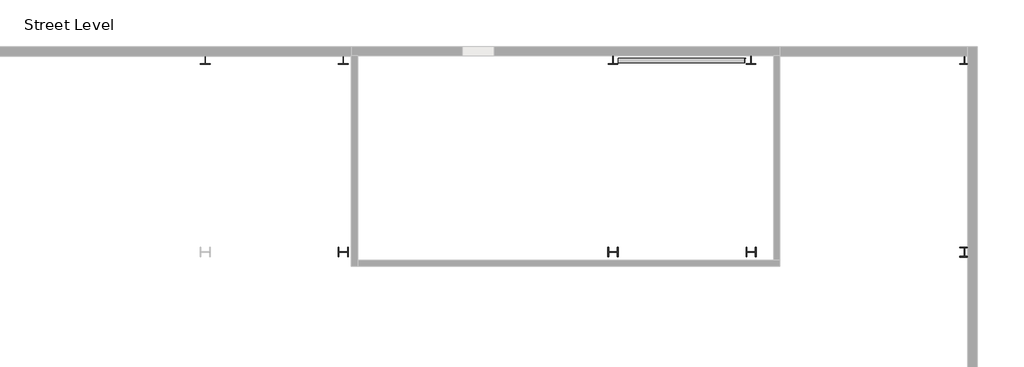
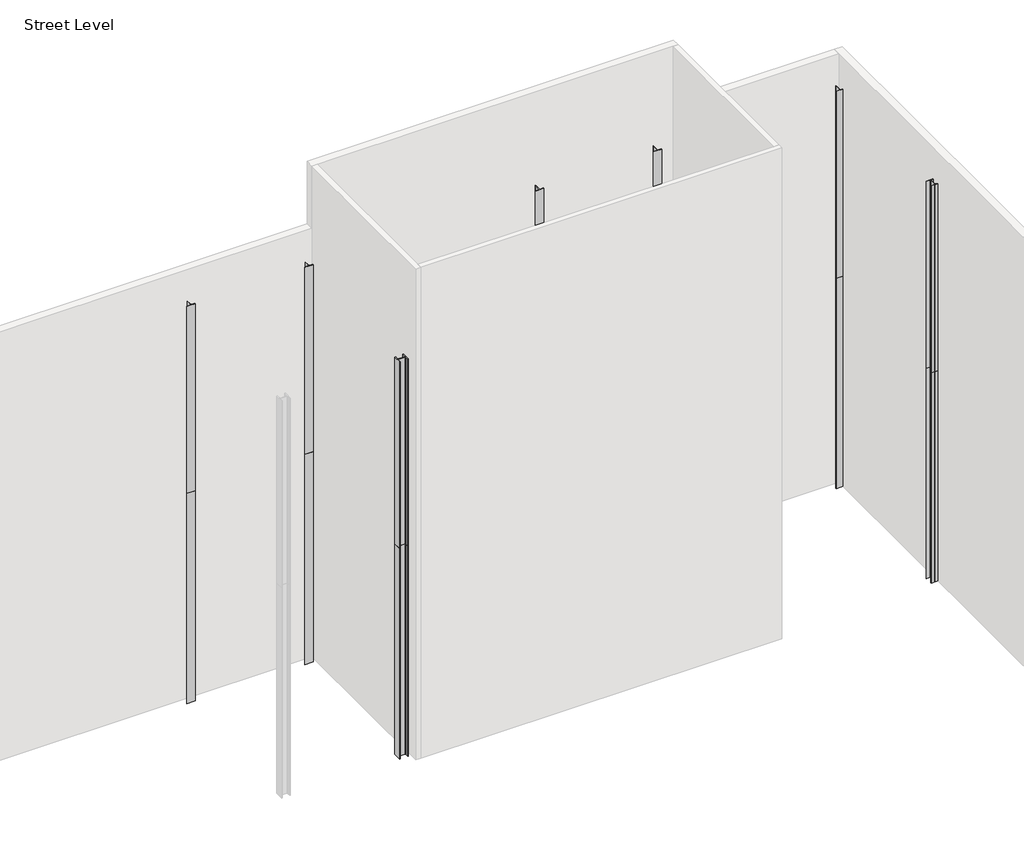
# One storey, part 3 of 3: 9 columns, 1 member.
"""IFC4 building model written with IfcOpenShell, lengths in millimetres."""

import ifcopenshell
import ifcopenshell.guid

model = None  # the IFC model being written
_history = None  # IfcOwnerHistory: only IFC2X3 demands one
_inside = {}  # id of a spatial element -> (the spatial element, [elements in it])
_under = {}  # id of a project, library or spatial element -> (it, [spatial elements below it])
_declared = {}  # id of a project -> (the project, [libraries it declares])
_typed = {}  # id of a type object -> (the type object, [elements of that type])
_made_of = {}  # id of a material, layer set ... -> (it, [elements and type objects made of it])


def new_model(schema):
    """Start an empty IFC model of exactly this schema.

    Asked for "IFC4X3", IfcOpenShell would pick the latest addendum, in which some entities
    have other attributes; the version numbers below select the first issue.
    IFC2X3 requires an IfcOwnerHistory on every rooted entity: one is made here for all.
    """
    global model, _history
    if schema == "IFC4X3":
        model = ifcopenshell.file(schema_version=(4, 3, 0, 0))
    else:
        model = ifcopenshell.file(schema=schema)
    _inside.clear()
    _under.clear()
    _declared.clear()
    _typed.clear()
    _made_of.clear()
    _history = None
    if model.schema == "IFC2X3":
        org = make("IfcOrganization", Name="unknown")
        user = make(
            "IfcPersonAndOrganization",
            ThePerson=make("IfcPerson", FamilyName="unknown"),
            TheOrganization=org,
        )
        app = make(
            "IfcApplication",
            ApplicationDeveloper=org,
            Version="unknown",
            ApplicationFullName="unknown",
            ApplicationIdentifier="unknown",
        )
        _history = make(
            "IfcOwnerHistory",
            OwningUser=user,
            OwningApplication=app,
            ChangeAction="ADDED",
            CreationDate=0,
        )
    return model


def make(cls, **values):
    """One entity of the class cls with the attributes given. An attribute that is None is left unset."""
    return model.create_entity(
        cls, **{name: value for name, value in values.items() if value is not None}
    )


def rooted(cls, **values):
    """An entity with a GlobalId (a new one), such as an element, a storey or a relation."""
    return make(cls, GlobalId=ifcopenshell.guid.new(), OwnerHistory=_history, **values)


def si_unit(unit_type, name, prefix=None):
    """IfcSIUnit, for example si_unit("LENGTHUNIT", "METRE", prefix="MILLI")."""
    return make("IfcSIUnit", UnitType=unit_type, Prefix=prefix, Name=name)


def assignment(units):
    """IfcUnitAssignment: the units of a project."""
    return None if units is None else make("IfcUnitAssignment", Units=units)


def point(xyz):
    """IfcCartesianPoint."""
    return None if xyz is None else make("IfcCartesianPoint", Coordinates=xyz)


def direction(xyz):
    """IfcDirection."""
    return None if xyz is None else make("IfcDirection", DirectionRatios=xyz)


def frame(location, z_axis=None, x_axis=None):
    """IfcAxis2Placement3D, a coordinate frame: its origin and axes. An axis left out is left unset."""
    return make(
        "IfcAxis2Placement3D",
        Location=point(location),
        Axis=direction(z_axis),
        RefDirection=direction(x_axis),
    )


def frame_2d(location, x_axis=None):
    """IfcAxis2Placement2D, a coordinate frame in the plane: its origin and x axis."""
    return make(
        "IfcAxis2Placement2D", Location=point(location), RefDirection=direction(x_axis)
    )


def origin():
    """The frame at (0, 0, 0) with its axes left unset."""
    return frame((0.0, 0.0, 0.0))


def place(relative_to, where):
    """IfcLocalPlacement: puts the frame where relative to a parent placement (None: the world)."""
    return make(
        "IfcLocalPlacement", PlacementRelTo=relative_to, RelativePlacement=where
    )


def context(
    kind, dimensions, precision=None, world=None, true_north=None, identifier=None
):
    """IfcGeometricRepresentationContext, for example the 3D "Model" context."""
    return make(
        "IfcGeometricRepresentationContext",
        ContextIdentifier=identifier,
        ContextType=kind,
        CoordinateSpaceDimension=dimensions,
        Precision=precision,
        WorldCoordinateSystem=world,
        TrueNorth=true_north,
    )


def project(units=None, contexts=None):
    """IfcProject with its units and contexts."""
    return rooted(
        "IfcProject",
        Name="project",
        RepresentationContexts=contexts,
        UnitsInContext=assignment(units),
    )


def spatial(cls, under=None, at=None, **own):
    """A site, building, storey or space (cls), placed at a placement, below another one or the project."""
    s = rooted(cls, ObjectPlacement=at, **own)
    if under is not None:
        _under.setdefault(under.id(), (under, []))[1].append(s)
    return s


def polyline(points):
    """IfcPolyline through the points."""
    return make("IfcPolyline", Points=[point(p) for p in points])


def circle_curve(where, radius):
    """IfcCircle in the frame where."""
    return make("IfcCircle", Position=where, Radius=radius)


def trimmed(basis, trim1, trim2, sense, master):
    """IfcTrimmedCurve: the piece of a basis curve between two trims."""
    return make(
        "IfcTrimmedCurve",
        BasisCurve=basis,
        Trim1=trim1,
        Trim2=trim2,
        SenseAgreement=sense,
        MasterRepresentation=master,
    )


def segment(curve, same_sense, transition):
    """IfcCompositeCurveSegment."""
    return make(
        "IfcCompositeCurveSegment",
        Transition=transition,
        SameSense=same_sense,
        ParentCurve=curve,
    )


def composite_curve(segments, self_intersect=None):
    """IfcCompositeCurve: segments joined end to end."""
    return make("IfcCompositeCurve", Segments=segments, SelfIntersect=self_intersect)


def outline(outer, holes=None, kind="AREA"):
    """IfcArbitraryClosedProfileDef: a profile drawn as a closed curve; with holes, ...WithVoids."""
    if holes is None:
        return make("IfcArbitraryClosedProfileDef", ProfileType=kind, OuterCurve=outer)
    return make(
        "IfcArbitraryProfileDefWithVoids",
        ProfileType=kind,
        OuterCurve=outer,
        InnerCurves=holes,
    )


def extrude(swept, where, along, depth):
    """IfcExtrudedAreaSolid: the profile swept, set in the frame where, extruded along a direction by depth."""
    return make(
        "IfcExtrudedAreaSolid",
        SweptArea=swept,
        Position=where,
        ExtrudedDirection=direction(along),
        Depth=depth,
    )


def shape(context_of_items, identifier, shape_type, items):
    """IfcShapeRepresentation: the items that make up one representation, for example the "Body"."""
    return make(
        "IfcShapeRepresentation",
        ContextOfItems=context_of_items,
        RepresentationIdentifier=identifier,
        RepresentationType=shape_type,
        Items=items,
    )


def source(mapping_origin, context_of_items, identifier, shape_type, items):
    """IfcRepresentationMap: a shape defined once, which mapped items show again and again."""
    return make(
        "IfcRepresentationMap",
        MappingOrigin=mapping_origin,
        MappedRepresentation=shape(context_of_items, identifier, shape_type, items),
    )


def transform(
    local_origin,
    x_axis=None,
    y_axis=None,
    z_axis=None,
    scale=None,
    scale2=None,
    scale3=None,
    uniform=True,
):
    """IfcCartesianTransformationOperator3D, or its non-uniform kind. x_axis, y_axis, z_axis: its Axis1, 2, 3."""
    if uniform:
        return make(
            "IfcCartesianTransformationOperator3D",
            Axis1=direction(x_axis),
            Axis2=direction(y_axis),
            LocalOrigin=point(local_origin),
            Scale=scale,
            Axis3=direction(z_axis),
        )
    return make(
        "IfcCartesianTransformationOperator3DnonUniform",
        Axis1=direction(x_axis),
        Axis2=direction(y_axis),
        LocalOrigin=point(local_origin),
        Scale=scale,
        Axis3=direction(z_axis),
        Scale2=scale2,
        Scale3=scale3,
    )


def mapped(mapping_source, mapping_target):
    """IfcMappedItem: shows the shape of a source again, moved by a transform."""
    return make(
        "IfcMappedItem", MappingSource=mapping_source, MappingTarget=mapping_target
    )


def made_of(thing, what):
    """Note that an element or type object is made of a material, layer set ...; save() writes the relation."""
    if what is not None:
        _made_of.setdefault(what.id(), (what, []))[1].append(thing)
    return thing


def element(
    cls,
    number,
    at=None,
    inside=None,
    cuts=None,
    type_object=None,
    material=None,
    context=None,
    identifier="Body",
    shape_type=None,
    held_by="IfcProductDefinitionShape",
    body=None,
    shapes=None,
    **own,
):
    """One element of the class cls, such as IfcWall. Its Tag is "e" and its number.

    at: its placement. inside: the storey or other place that contains it. cuts: it is an
    opening in that element (IfcRelVoidsElement). A single representation is given by context,
    identifier, shape_type and body (its items); several are given by shapes. held_by: the class
    of the entity that holds the representations. save() writes the other relations.
    """
    e = rooted(cls, Tag="e%d" % number, ObjectPlacement=at, **own)
    if body is not None:
        shapes = [shape(context, identifier, shape_type, body)]
    if shapes is not None:
        e.Representation = make(held_by, Representations=shapes)
    if inside is not None:
        _inside.setdefault(inside.id(), (inside, []))[1].append(e)
    if cuts is not None:
        rooted(
            "IfcRelVoidsElement", RelatingBuildingElement=cuts, RelatedOpeningElement=e
        )
    if type_object is not None:
        _typed.setdefault(type_object.id(), (type_object, []))[1].append(e)
    return made_of(e, material)


def aggregate(whole, parts):
    """IfcRelAggregates: a whole, such as a stair, and the parts it consists of."""
    return rooted("IfcRelAggregates", RelatingObject=whole, RelatedObjects=parts)


def save(model, path):
    """Write the relations noted so far, then the file.

    IfcRelAggregates (storeys below a building ...), IfcRelContainedInSpatialStructure (elements
    in a storey), IfcRelDefinesByType, IfcRelAssociatesMaterial and IfcRelDeclares: one each for
    every whole, place, type object, material and project.
    """
    for whole, parts in _under.values():
        aggregate(whole, parts)
    for where, things in _inside.values():
        rooted(
            "IfcRelContainedInSpatialStructure",
            RelatedElements=things,
            RelatingStructure=where,
        )
    for kind, things in _typed.values():
        rooted("IfcRelDefinesByType", RelatedObjects=things, RelatingType=kind)
    for what, things in _made_of.values():
        rooted("IfcRelAssociatesMaterial", RelatedObjects=things, RelatingMaterial=what)
    for by, libraries in _declared.values():
        rooted("IfcRelDeclares", RelatingContext=by, RelatedDefinitions=libraries)
    model.write(path)


def l_angle_l6x6x3_8_1e5b70da(model_context):
    return source(origin(), model_context, "Body", "SweptSolid", [
        extrude(outline(composite_curve([segment(polyline([(41.148, 41.148), (41.148, -111.252)]), True, "CONTINUOUS"), segment(trimmed(circle_curve(frame_2d((41.148, -101.727)), 9.525), [point((41.148, -111.252))], [point((31.623, -101.727))], False, "CARTESIAN"), True, "CONTINUOUS"), segment(polyline([(31.623, -101.727), (31.623, 22.098)]), True, "CONTINUOUS"), segment(trimmed(circle_curve(frame_2d((22.098, 22.098)), 9.525), [point((31.623, 22.098))], [point((22.098, 31.623))], True, "CARTESIAN"), True, "CONTINUOUS"), segment(polyline([(22.098, 31.623), (-101.727, 31.623)]), True, "CONTINUOUS"), segment(trimmed(circle_curve(frame_2d((-101.727, 41.148)), 9.525), [point((-101.727, 31.623))], [point((-111.252, 41.148))], False, "CARTESIAN"), True, "CONTINUOUS"), segment(polyline([(-111.252, 41.148), (41.148, 41.148)]), True, "CONTINUOUS")], self_intersect=False)), frame((-2053.4214347, 0.0, 0.0), z_axis=(1.0, 0.0, 0.0), x_axis=(0.0, 1.0, 0.0)), (0.0, 0.0, 1.0), 4092.1699392),
    ])


model = new_model("IFC4")

# Units and contexts
model_context = context("Model", 3, world=origin())
ifc_project = project(units=[si_unit("LENGTHUNIT", "METRE", prefix="MILLI")], contexts=[model_context])

# Site, building, storey
site = spatial("IfcSite", under=ifc_project)
building = spatial("IfcBuilding", under=site)
storey = spatial("IfcBuildingStorey", under=building, Name="Street Level", Elevation=-914.4)

# Columns
placement = place(None, origin())
element("IfcColumn", 1, ObjectType="W-Wide Flange-Column : W12X87", at=placement, inside=storey, context=model_context, shape_type="SweptSolid", body=[
    extrude(outline(composite_curve([segment(polyline([(-5274.2622732, 2940.2315304), (-5294.8362732, 2940.2315304), (-5294.8362732, 3065.0725304)]), True, "CONTINUOUS"), segment(trimmed(circle_curve(frame_2d((-5317.1247732, 3065.0725304)), 22.2885), [point((-5294.8362732, 3065.0725304))], [point((-5317.1247732, 3087.3610304))], True, "CARTESIAN"), True, "CONTINUOUS"), segment(polyline([(-5317.1247732, 3087.3610304), (-5548.8997732, 3087.3610304)]), True, "CONTINUOUS"), segment(trimmed(circle_curve(frame_2d((-5548.8997732, 3065.0725304)), 22.2885), [point((-5548.8997732, 3087.3610304))], [point((-5571.1882732, 3065.0725304))], True, "CARTESIAN"), True, "CONTINUOUS"), segment(polyline([(-5571.1882732, 3065.0725304), (-5571.1882732, 2940.2315304), (-5591.7622732, 2940.2315304), (-5591.7622732, 3247.5715304), (-5571.1882732, 3247.5715304), (-5571.1882732, 3122.7305304)]), True, "CONTINUOUS"), segment(trimmed(circle_curve(frame_2d((-5548.8997732, 3122.7305304)), 22.2885), [point((-5571.1882732, 3122.7305304))], [point((-5548.8997732, 3100.4420304))], True, "CARTESIAN"), True, "CONTINUOUS"), segment(polyline([(-5548.8997732, 3100.4420304), (-5317.1247732, 3100.4420304)]), True, "CONTINUOUS"), segment(trimmed(circle_curve(frame_2d((-5317.1247732, 3122.7305304)), 22.2885), [point((-5317.1247732, 3100.4420304))], [point((-5294.8362732, 3122.7305304))], True, "CARTESIAN"), True, "CONTINUOUS"), segment(polyline([(-5294.8362732, 3122.7305304), (-5294.8362732, 3247.5715304), (-5274.2622732, 3247.5715304), (-5274.2622732, 2940.2315304)]), True, "CONTINUOUS")], self_intersect=False)), frame((0.0, 0.0, 7315.2), z_axis=(0.0, 0.0, 1.0), x_axis=(1.0, 0.0, 0.0)), (0.0, 0.0, 1.0), 7315.2),
    extrude(outline(composite_curve([segment(polyline([(-5274.2622732, 2940.2315304), (-5294.8362732, 2940.2315304), (-5294.8362732, 3065.0725304)]), True, "CONTINUOUS"), segment(trimmed(circle_curve(frame_2d((-5317.1247732, 3065.0725304)), 22.2885), [point((-5294.8362732, 3065.0725304))], [point((-5317.1247732, 3087.3610304))], True, "CARTESIAN"), True, "CONTINUOUS"), segment(polyline([(-5317.1247732, 3087.3610304), (-5548.8997732, 3087.3610304)]), True, "CONTINUOUS"), segment(trimmed(circle_curve(frame_2d((-5548.8997732, 3065.0725304)), 22.2885), [point((-5548.8997732, 3087.3610304))], [point((-5571.1882732, 3065.0725304))], True, "CARTESIAN"), True, "CONTINUOUS"), segment(polyline([(-5571.1882732, 3065.0725304), (-5571.1882732, 2940.2315304), (-5591.7622732, 2940.2315304), (-5591.7622732, 3247.5715304), (-5571.1882732, 3247.5715304), (-5571.1882732, 3122.7305304)]), True, "CONTINUOUS"), segment(trimmed(circle_curve(frame_2d((-5548.8997732, 3122.7305304)), 22.2885), [point((-5571.1882732, 3122.7305304))], [point((-5548.8997732, 3100.4420304))], True, "CARTESIAN"), True, "CONTINUOUS"), segment(polyline([(-5548.8997732, 3100.4420304), (-5317.1247732, 3100.4420304)]), True, "CONTINUOUS"), segment(trimmed(circle_curve(frame_2d((-5317.1247732, 3122.7305304)), 22.2885), [point((-5317.1247732, 3100.4420304))], [point((-5294.8362732, 3122.7305304))], True, "CARTESIAN"), True, "CONTINUOUS"), segment(polyline([(-5294.8362732, 3122.7305304), (-5294.8362732, 3247.5715304), (-5274.2622732, 3247.5715304), (-5274.2622732, 2940.2315304)]), True, "CONTINUOUS")], self_intersect=False)), frame((0.0, 0.0, -914.4), z_axis=(0.0, 0.0, 1.0), x_axis=(1.0, 0.0, 0.0)), (0.0, 0.0, 1.0), 8229.6),
])
element("IfcColumn", 2, ObjectType="W-Wide Flange-Column : W12X87", at=placement, inside=storey, context=model_context, shape_type="SweptSolid", body=[
    extrude(outline(composite_curve([segment(polyline([(3260.1377268, 2940.2315304), (3239.5637268, 2940.2315304), (3239.5637268, 3065.0725304)]), True, "CONTINUOUS"), segment(trimmed(circle_curve(frame_2d((3217.2752268, 3065.0725304)), 22.2885), [point((3239.5637268, 3065.0725304))], [point((3217.2752268, 3087.3610304))], True, "CARTESIAN"), True, "CONTINUOUS"), segment(polyline([(3217.2752268, 3087.3610304), (2985.5002268, 3087.3610304)]), True, "CONTINUOUS"), segment(trimmed(circle_curve(frame_2d((2985.5002268, 3065.0725304)), 22.2885), [point((2985.5002268, 3087.3610304))], [point((2963.2117268, 3065.0725304))], True, "CARTESIAN"), True, "CONTINUOUS"), segment(polyline([(2963.2117268, 3065.0725304), (2963.2117268, 2940.2315304), (2942.6377268, 2940.2315304), (2942.6377268, 3247.5715304), (2963.2117268, 3247.5715304), (2963.2117268, 3122.7305304)]), True, "CONTINUOUS"), segment(trimmed(circle_curve(frame_2d((2985.5002268, 3122.7305304)), 22.2885), [point((2963.2117268, 3122.7305304))], [point((2985.5002268, 3100.4420304))], True, "CARTESIAN"), True, "CONTINUOUS"), segment(polyline([(2985.5002268, 3100.4420304), (3217.2752268, 3100.4420304)]), True, "CONTINUOUS"), segment(trimmed(circle_curve(frame_2d((3217.2752268, 3122.7305304)), 22.2885), [point((3217.2752268, 3100.4420304))], [point((3239.5637268, 3122.7305304))], True, "CARTESIAN"), True, "CONTINUOUS"), segment(polyline([(3239.5637268, 3122.7305304), (3239.5637268, 3247.5715304), (3260.1377268, 3247.5715304), (3260.1377268, 2940.2315304)]), True, "CONTINUOUS")], self_intersect=False)), frame((0.0, 0.0, 7315.2), z_axis=(0.0, 0.0, 1.0), x_axis=(1.0, 0.0, 0.0)), (0.0, 0.0, 1.0), 7315.2),
    extrude(outline(composite_curve([segment(polyline([(3260.1377268, 2940.2315304), (3239.5637268, 2940.2315304), (3239.5637268, 3065.0725304)]), True, "CONTINUOUS"), segment(trimmed(circle_curve(frame_2d((3217.2752268, 3065.0725304)), 22.2885), [point((3239.5637268, 3065.0725304))], [point((3217.2752268, 3087.3610304))], True, "CARTESIAN"), True, "CONTINUOUS"), segment(polyline([(3217.2752268, 3087.3610304), (2985.5002268, 3087.3610304)]), True, "CONTINUOUS"), segment(trimmed(circle_curve(frame_2d((2985.5002268, 3065.0725304)), 22.2885), [point((2985.5002268, 3087.3610304))], [point((2963.2117268, 3065.0725304))], True, "CARTESIAN"), True, "CONTINUOUS"), segment(polyline([(2963.2117268, 3065.0725304), (2963.2117268, 2940.2315304), (2942.6377268, 2940.2315304), (2942.6377268, 3247.5715304), (2963.2117268, 3247.5715304), (2963.2117268, 3122.7305304)]), True, "CONTINUOUS"), segment(trimmed(circle_curve(frame_2d((2985.5002268, 3122.7305304)), 22.2885), [point((2963.2117268, 3122.7305304))], [point((2985.5002268, 3100.4420304))], True, "CARTESIAN"), True, "CONTINUOUS"), segment(polyline([(2985.5002268, 3100.4420304), (3217.2752268, 3100.4420304)]), True, "CONTINUOUS"), segment(trimmed(circle_curve(frame_2d((3217.2752268, 3122.7305304)), 22.2885), [point((3217.2752268, 3100.4420304))], [point((3239.5637268, 3122.7305304))], True, "CARTESIAN"), True, "CONTINUOUS"), segment(polyline([(3239.5637268, 3122.7305304), (3239.5637268, 3247.5715304), (3260.1377268, 3247.5715304), (3260.1377268, 2940.2315304)]), True, "CONTINUOUS")], self_intersect=False)), frame((0.0, 0.0, -914.4), z_axis=(0.0, 0.0, 1.0), x_axis=(1.0, 0.0, 0.0)), (0.0, 0.0, 1.0), 8229.6),
])
element("IfcColumn", 3, ObjectType="W-Wide Flange-Column : W12X87", at=placement, inside=storey, context=model_context, shape_type="SweptSolid", body=[
    extrude(outline(composite_curve([segment(polyline([(7628.9377268, 2940.2315304), (7608.3637268, 2940.2315304), (7608.3637268, 3065.0725304)]), True, "CONTINUOUS"), segment(trimmed(circle_curve(frame_2d((7586.0752268, 3065.0725304)), 22.2885), [point((7608.3637268, 3065.0725304))], [point((7586.0752268, 3087.3610304))], True, "CARTESIAN"), True, "CONTINUOUS"), segment(polyline([(7586.0752268, 3087.3610304), (7354.3002268, 3087.3610304)]), True, "CONTINUOUS"), segment(trimmed(circle_curve(frame_2d((7354.3002268, 3065.0725304)), 22.2885), [point((7354.3002268, 3087.3610304))], [point((7332.0117268, 3065.0725304))], True, "CARTESIAN"), True, "CONTINUOUS"), segment(polyline([(7332.0117268, 3065.0725304), (7332.0117268, 2940.2315304), (7311.4377268, 2940.2315304), (7311.4377268, 3247.5715304), (7332.0117268, 3247.5715304), (7332.0117268, 3122.7305304)]), True, "CONTINUOUS"), segment(trimmed(circle_curve(frame_2d((7354.3002268, 3122.7305304)), 22.2885), [point((7332.0117268, 3122.7305304))], [point((7354.3002268, 3100.4420304))], True, "CARTESIAN"), True, "CONTINUOUS"), segment(polyline([(7354.3002268, 3100.4420304), (7586.0752268, 3100.4420304)]), True, "CONTINUOUS"), segment(trimmed(circle_curve(frame_2d((7586.0752268, 3122.7305304)), 22.2885), [point((7586.0752268, 3100.4420304))], [point((7608.3637268, 3122.7305304))], True, "CARTESIAN"), True, "CONTINUOUS"), segment(polyline([(7608.3637268, 3122.7305304), (7608.3637268, 3247.5715304), (7628.9377268, 3247.5715304), (7628.9377268, 2940.2315304)]), True, "CONTINUOUS")], self_intersect=False)), frame((0.0, 0.0, 7315.2), z_axis=(0.0, 0.0, 1.0), x_axis=(1.0, 0.0, 0.0)), (0.0, 0.0, 1.0), 7315.2),
    extrude(outline(composite_curve([segment(polyline([(7628.9377268, 2940.2315304), (7608.3637268, 2940.2315304), (7608.3637268, 3065.0725304)]), True, "CONTINUOUS"), segment(trimmed(circle_curve(frame_2d((7586.0752268, 3065.0725304)), 22.2885), [point((7608.3637268, 3065.0725304))], [point((7586.0752268, 3087.3610304))], True, "CARTESIAN"), True, "CONTINUOUS"), segment(polyline([(7586.0752268, 3087.3610304), (7354.3002268, 3087.3610304)]), True, "CONTINUOUS"), segment(trimmed(circle_curve(frame_2d((7354.3002268, 3065.0725304)), 22.2885), [point((7354.3002268, 3087.3610304))], [point((7332.0117268, 3065.0725304))], True, "CARTESIAN"), True, "CONTINUOUS"), segment(polyline([(7332.0117268, 3065.0725304), (7332.0117268, 2940.2315304), (7311.4377268, 2940.2315304), (7311.4377268, 3247.5715304), (7332.0117268, 3247.5715304), (7332.0117268, 3122.7305304)]), True, "CONTINUOUS"), segment(trimmed(circle_curve(frame_2d((7354.3002268, 3122.7305304)), 22.2885), [point((7332.0117268, 3122.7305304))], [point((7354.3002268, 3100.4420304))], True, "CARTESIAN"), True, "CONTINUOUS"), segment(polyline([(7354.3002268, 3100.4420304), (7586.0752268, 3100.4420304)]), True, "CONTINUOUS"), segment(trimmed(circle_curve(frame_2d((7586.0752268, 3122.7305304)), 22.2885), [point((7586.0752268, 3100.4420304))], [point((7608.3637268, 3122.7305304))], True, "CARTESIAN"), True, "CONTINUOUS"), segment(polyline([(7608.3637268, 3122.7305304), (7608.3637268, 3247.5715304), (7628.9377268, 3247.5715304), (7628.9377268, 2940.2315304)]), True, "CONTINUOUS")], self_intersect=False)), frame((0.0, 0.0, -914.4), z_axis=(0.0, 0.0, 1.0), x_axis=(1.0, 0.0, 0.0)), (0.0, 0.0, 1.0), 8229.6),
])
element("IfcColumn", 4, ObjectType="W-Wide Flange-Column : W12X87", at=placement, inside=storey, context=model_context, shape_type="SweptSolid", body=[
    extrude(outline(composite_curve([segment(polyline([(-9648.1422732, 9348.6515304), (-9648.1422732, 9328.0775304), (-9772.9832732, 9328.0775304)]), True, "CONTINUOUS"), segment(trimmed(circle_curve(frame_2d((-9772.9832732, 9305.7890304)), 22.2885), [point((-9772.9832732, 9328.0775304))], [point((-9795.2717732, 9305.7890304))], True, "CARTESIAN"), True, "CONTINUOUS"), segment(polyline([(-9795.2717732, 9305.7890304), (-9795.2717732, 9074.0140304)]), True, "CONTINUOUS"), segment(trimmed(circle_curve(frame_2d((-9772.9832732, 9074.0140304)), 22.2885), [point((-9795.2717732, 9074.0140304))], [point((-9772.9832732, 9051.7255304))], True, "CARTESIAN"), True, "CONTINUOUS"), segment(polyline([(-9772.9832732, 9051.7255304), (-9648.1422732, 9051.7255304), (-9648.1422732, 9031.1515304), (-9955.4822732, 9031.1515304), (-9955.4822732, 9051.7255304), (-9830.6412732, 9051.7255304)]), True, "CONTINUOUS"), segment(trimmed(circle_curve(frame_2d((-9830.6412732, 9074.0140304)), 22.2885), [point((-9830.6412732, 9051.7255304))], [point((-9808.3527732, 9074.0140304))], True, "CARTESIAN"), True, "CONTINUOUS"), segment(polyline([(-9808.3527732, 9074.0140304), (-9808.3527732, 9305.7890304)]), True, "CONTINUOUS"), segment(trimmed(circle_curve(frame_2d((-9830.6412732, 9305.7890304)), 22.2885), [point((-9808.3527732, 9305.7890304))], [point((-9830.6412732, 9328.0775304))], True, "CARTESIAN"), True, "CONTINUOUS"), segment(polyline([(-9830.6412732, 9328.0775304), (-9955.4822732, 9328.0775304), (-9955.4822732, 9348.6515304), (-9648.1422732, 9348.6515304)]), True, "CONTINUOUS")], self_intersect=False)), frame((0.0, 0.0, 7315.2), z_axis=(0.0, 0.0, 1.0), x_axis=(1.0, 0.0, 0.0)), (0.0, 0.0, 1.0), 7315.2),
    extrude(outline(composite_curve([segment(polyline([(-9648.1422732, 9348.6515304), (-9648.1422732, 9328.0775304), (-9772.9832732, 9328.0775304)]), True, "CONTINUOUS"), segment(trimmed(circle_curve(frame_2d((-9772.9832732, 9305.7890304)), 22.2885), [point((-9772.9832732, 9328.0775304))], [point((-9795.2717732, 9305.7890304))], True, "CARTESIAN"), True, "CONTINUOUS"), segment(polyline([(-9795.2717732, 9305.7890304), (-9795.2717732, 9074.0140304)]), True, "CONTINUOUS"), segment(trimmed(circle_curve(frame_2d((-9772.9832732, 9074.0140304)), 22.2885), [point((-9795.2717732, 9074.0140304))], [point((-9772.9832732, 9051.7255304))], True, "CARTESIAN"), True, "CONTINUOUS"), segment(polyline([(-9772.9832732, 9051.7255304), (-9648.1422732, 9051.7255304), (-9648.1422732, 9031.1515304), (-9955.4822732, 9031.1515304), (-9955.4822732, 9051.7255304), (-9830.6412732, 9051.7255304)]), True, "CONTINUOUS"), segment(trimmed(circle_curve(frame_2d((-9830.6412732, 9074.0140304)), 22.2885), [point((-9830.6412732, 9051.7255304))], [point((-9808.3527732, 9074.0140304))], True, "CARTESIAN"), True, "CONTINUOUS"), segment(polyline([(-9808.3527732, 9074.0140304), (-9808.3527732, 9305.7890304)]), True, "CONTINUOUS"), segment(trimmed(circle_curve(frame_2d((-9830.6412732, 9305.7890304)), 22.2885), [point((-9808.3527732, 9305.7890304))], [point((-9830.6412732, 9328.0775304))], True, "CARTESIAN"), True, "CONTINUOUS"), segment(polyline([(-9830.6412732, 9328.0775304), (-9955.4822732, 9328.0775304), (-9955.4822732, 9348.6515304), (-9648.1422732, 9348.6515304)]), True, "CONTINUOUS")], self_intersect=False)), frame((0.0, 0.0, -914.4), z_axis=(0.0, 0.0, 1.0), x_axis=(1.0, 0.0, 0.0)), (0.0, 0.0, 1.0), 8229.6),
])
element("IfcColumn", 5, ObjectType="W-Wide Flange-Column : W12X87", at=placement, inside=storey, context=model_context, shape_type="SweptSolid", body=[
    extrude(outline(composite_curve([segment(polyline([(-5279.3422732, 9348.6515304), (-5279.3422732, 9328.0775304), (-5404.1832732, 9328.0775304)]), True, "CONTINUOUS"), segment(trimmed(circle_curve(frame_2d((-5404.1832732, 9305.7890304)), 22.2885), [point((-5404.1832732, 9328.0775304))], [point((-5426.4717732, 9305.7890304))], True, "CARTESIAN"), True, "CONTINUOUS"), segment(polyline([(-5426.4717732, 9305.7890304), (-5426.4717732, 9074.0140304)]), True, "CONTINUOUS"), segment(trimmed(circle_curve(frame_2d((-5404.1832732, 9074.0140304)), 22.2885), [point((-5426.4717732, 9074.0140304))], [point((-5404.1832732, 9051.7255304))], True, "CARTESIAN"), True, "CONTINUOUS"), segment(polyline([(-5404.1832732, 9051.7255304), (-5279.3422732, 9051.7255304), (-5279.3422732, 9031.1515304), (-5586.6822732, 9031.1515304), (-5586.6822732, 9051.7255304), (-5461.8412732, 9051.7255304)]), True, "CONTINUOUS"), segment(trimmed(circle_curve(frame_2d((-5461.8412732, 9074.0140304)), 22.2885), [point((-5461.8412732, 9051.7255304))], [point((-5439.5527732, 9074.0140304))], True, "CARTESIAN"), True, "CONTINUOUS"), segment(polyline([(-5439.5527732, 9074.0140304), (-5439.5527732, 9305.7890304)]), True, "CONTINUOUS"), segment(trimmed(circle_curve(frame_2d((-5461.8412732, 9305.7890304)), 22.2885), [point((-5439.5527732, 9305.7890304))], [point((-5461.8412732, 9328.0775304))], True, "CARTESIAN"), True, "CONTINUOUS"), segment(polyline([(-5461.8412732, 9328.0775304), (-5586.6822732, 9328.0775304), (-5586.6822732, 9348.6515304), (-5279.3422732, 9348.6515304)]), True, "CONTINUOUS")], self_intersect=False)), frame((0.0, 0.0, 7315.2), z_axis=(0.0, 0.0, 1.0), x_axis=(1.0, 0.0, 0.0)), (0.0, 0.0, 1.0), 7315.2),
    extrude(outline(composite_curve([segment(polyline([(-5279.3422732, 9348.6515304), (-5279.3422732, 9328.0775304), (-5404.1832732, 9328.0775304)]), True, "CONTINUOUS"), segment(trimmed(circle_curve(frame_2d((-5404.1832732, 9305.7890304)), 22.2885), [point((-5404.1832732, 9328.0775304))], [point((-5426.4717732, 9305.7890304))], True, "CARTESIAN"), True, "CONTINUOUS"), segment(polyline([(-5426.4717732, 9305.7890304), (-5426.4717732, 9074.0140304)]), True, "CONTINUOUS"), segment(trimmed(circle_curve(frame_2d((-5404.1832732, 9074.0140304)), 22.2885), [point((-5426.4717732, 9074.0140304))], [point((-5404.1832732, 9051.7255304))], True, "CARTESIAN"), True, "CONTINUOUS"), segment(polyline([(-5404.1832732, 9051.7255304), (-5279.3422732, 9051.7255304), (-5279.3422732, 9031.1515304), (-5586.6822732, 9031.1515304), (-5586.6822732, 9051.7255304), (-5461.8412732, 9051.7255304)]), True, "CONTINUOUS"), segment(trimmed(circle_curve(frame_2d((-5461.8412732, 9074.0140304)), 22.2885), [point((-5461.8412732, 9051.7255304))], [point((-5439.5527732, 9074.0140304))], True, "CARTESIAN"), True, "CONTINUOUS"), segment(polyline([(-5439.5527732, 9074.0140304), (-5439.5527732, 9305.7890304)]), True, "CONTINUOUS"), segment(trimmed(circle_curve(frame_2d((-5461.8412732, 9305.7890304)), 22.2885), [point((-5439.5527732, 9305.7890304))], [point((-5461.8412732, 9328.0775304))], True, "CARTESIAN"), True, "CONTINUOUS"), segment(polyline([(-5461.8412732, 9328.0775304), (-5586.6822732, 9328.0775304), (-5586.6822732, 9348.6515304), (-5279.3422732, 9348.6515304)]), True, "CONTINUOUS")], self_intersect=False)), frame((0.0, 0.0, -914.4), z_axis=(0.0, 0.0, 1.0), x_axis=(1.0, 0.0, 0.0)), (0.0, 0.0, 1.0), 8229.6),
])
element("IfcColumn", 6, ObjectType="W-Wide Flange-Column : W12X87", at=placement, inside=storey, context=model_context, shape_type="SweptSolid", body=[
    extrude(outline(composite_curve([segment(polyline([(3255.0577268, 9348.6515304), (3255.0577268, 9328.0775304), (3130.2167268, 9328.0775304)]), True, "CONTINUOUS"), segment(trimmed(circle_curve(frame_2d((3130.2167268, 9305.7890304)), 22.2885), [point((3130.2167268, 9328.0775304))], [point((3107.9282268, 9305.7890304))], True, "CARTESIAN"), True, "CONTINUOUS"), segment(polyline([(3107.9282268, 9305.7890304), (3107.9282268, 9074.0140304)]), True, "CONTINUOUS"), segment(trimmed(circle_curve(frame_2d((3130.2167268, 9074.0140304)), 22.2885), [point((3107.9282268, 9074.0140304))], [point((3130.2167268, 9051.7255304))], True, "CARTESIAN"), True, "CONTINUOUS"), segment(polyline([(3130.2167268, 9051.7255304), (3255.0577268, 9051.7255304), (3255.0577268, 9031.1515304), (2947.7177268, 9031.1515304), (2947.7177268, 9051.7255304), (3072.5587268, 9051.7255304)]), True, "CONTINUOUS"), segment(trimmed(circle_curve(frame_2d((3072.5587268, 9074.0140304)), 22.2885), [point((3072.5587268, 9051.7255304))], [point((3094.8472268, 9074.0140304))], True, "CARTESIAN"), True, "CONTINUOUS"), segment(polyline([(3094.8472268, 9074.0140304), (3094.8472268, 9305.7890304)]), True, "CONTINUOUS"), segment(trimmed(circle_curve(frame_2d((3072.5587268, 9305.7890304)), 22.2885), [point((3094.8472268, 9305.7890304))], [point((3072.5587268, 9328.0775304))], True, "CARTESIAN"), True, "CONTINUOUS"), segment(polyline([(3072.5587268, 9328.0775304), (2947.7177268, 9328.0775304), (2947.7177268, 9348.6515304), (3255.0577268, 9348.6515304)]), True, "CONTINUOUS")], self_intersect=False)), frame((0.0, 0.0, 7315.2), z_axis=(0.0, 0.0, 1.0), x_axis=(1.0, 0.0, 0.0)), (0.0, 0.0, 1.0), 7315.2),
    extrude(outline(composite_curve([segment(polyline([(3255.0577268, 9348.6515304), (3255.0577268, 9328.0775304), (3130.2167268, 9328.0775304)]), True, "CONTINUOUS"), segment(trimmed(circle_curve(frame_2d((3130.2167268, 9305.7890304)), 22.2885), [point((3130.2167268, 9328.0775304))], [point((3107.9282268, 9305.7890304))], True, "CARTESIAN"), True, "CONTINUOUS"), segment(polyline([(3107.9282268, 9305.7890304), (3107.9282268, 9074.0140304)]), True, "CONTINUOUS"), segment(trimmed(circle_curve(frame_2d((3130.2167268, 9074.0140304)), 22.2885), [point((3107.9282268, 9074.0140304))], [point((3130.2167268, 9051.7255304))], True, "CARTESIAN"), True, "CONTINUOUS"), segment(polyline([(3130.2167268, 9051.7255304), (3255.0577268, 9051.7255304), (3255.0577268, 9031.1515304), (2947.7177268, 9031.1515304), (2947.7177268, 9051.7255304), (3072.5587268, 9051.7255304)]), True, "CONTINUOUS"), segment(trimmed(circle_curve(frame_2d((3072.5587268, 9074.0140304)), 22.2885), [point((3072.5587268, 9051.7255304))], [point((3094.8472268, 9074.0140304))], True, "CARTESIAN"), True, "CONTINUOUS"), segment(polyline([(3094.8472268, 9074.0140304), (3094.8472268, 9305.7890304)]), True, "CONTINUOUS"), segment(trimmed(circle_curve(frame_2d((3072.5587268, 9305.7890304)), 22.2885), [point((3094.8472268, 9305.7890304))], [point((3072.5587268, 9328.0775304))], True, "CARTESIAN"), True, "CONTINUOUS"), segment(polyline([(3072.5587268, 9328.0775304), (2947.7177268, 9328.0775304), (2947.7177268, 9348.6515304), (3255.0577268, 9348.6515304)]), True, "CONTINUOUS")], self_intersect=False)), frame((0.0, 0.0, -914.4), z_axis=(0.0, 0.0, 1.0), x_axis=(1.0, 0.0, 0.0)), (0.0, 0.0, 1.0), 8229.6),
])
element("IfcColumn", 7, ObjectType="W-Wide Flange-Column : W12X87", at=placement, inside=storey, context=model_context, shape_type="SweptSolid", body=[
    extrude(outline(composite_curve([segment(polyline([(7623.8577268, 9348.6515304), (7623.8577268, 9328.0775304), (7499.0167268, 9328.0775304)]), True, "CONTINUOUS"), segment(trimmed(circle_curve(frame_2d((7499.0167268, 9305.7890304)), 22.2885), [point((7499.0167268, 9328.0775304))], [point((7476.7282268, 9305.7890304))], True, "CARTESIAN"), True, "CONTINUOUS"), segment(polyline([(7476.7282268, 9305.7890304), (7476.7282268, 9074.0140304)]), True, "CONTINUOUS"), segment(trimmed(circle_curve(frame_2d((7499.0167268, 9074.0140304)), 22.2885), [point((7476.7282268, 9074.0140304))], [point((7499.0167268, 9051.7255304))], True, "CARTESIAN"), True, "CONTINUOUS"), segment(polyline([(7499.0167268, 9051.7255304), (7623.8577268, 9051.7255304), (7623.8577268, 9031.1515304), (7316.5177268, 9031.1515304), (7316.5177268, 9051.7255304), (7441.3587268, 9051.7255304)]), True, "CONTINUOUS"), segment(trimmed(circle_curve(frame_2d((7441.3587268, 9074.0140304)), 22.2885), [point((7441.3587268, 9051.7255304))], [point((7463.6472268, 9074.0140304))], True, "CARTESIAN"), True, "CONTINUOUS"), segment(polyline([(7463.6472268, 9074.0140304), (7463.6472268, 9305.7890304)]), True, "CONTINUOUS"), segment(trimmed(circle_curve(frame_2d((7441.3587268, 9305.7890304)), 22.2885), [point((7463.6472268, 9305.7890304))], [point((7441.3587268, 9328.0775304))], True, "CARTESIAN"), True, "CONTINUOUS"), segment(polyline([(7441.3587268, 9328.0775304), (7316.5177268, 9328.0775304), (7316.5177268, 9348.6515304), (7623.8577268, 9348.6515304)]), True, "CONTINUOUS")], self_intersect=False)), frame((0.0, 0.0, 7315.2), z_axis=(0.0, 0.0, 1.0), x_axis=(1.0, 0.0, 0.0)), (0.0, 0.0, 1.0), 7315.2),
    extrude(outline(composite_curve([segment(polyline([(7623.8577268, 9348.6515304), (7623.8577268, 9328.0775304), (7499.0167268, 9328.0775304)]), True, "CONTINUOUS"), segment(trimmed(circle_curve(frame_2d((7499.0167268, 9305.7890304)), 22.2885), [point((7499.0167268, 9328.0775304))], [point((7476.7282268, 9305.7890304))], True, "CARTESIAN"), True, "CONTINUOUS"), segment(polyline([(7476.7282268, 9305.7890304), (7476.7282268, 9074.0140304)]), True, "CONTINUOUS"), segment(trimmed(circle_curve(frame_2d((7499.0167268, 9074.0140304)), 22.2885), [point((7476.7282268, 9074.0140304))], [point((7499.0167268, 9051.7255304))], True, "CARTESIAN"), True, "CONTINUOUS"), segment(polyline([(7499.0167268, 9051.7255304), (7623.8577268, 9051.7255304), (7623.8577268, 9031.1515304), (7316.5177268, 9031.1515304), (7316.5177268, 9051.7255304), (7441.3587268, 9051.7255304)]), True, "CONTINUOUS"), segment(trimmed(circle_curve(frame_2d((7441.3587268, 9074.0140304)), 22.2885), [point((7441.3587268, 9051.7255304))], [point((7463.6472268, 9074.0140304))], True, "CARTESIAN"), True, "CONTINUOUS"), segment(polyline([(7463.6472268, 9074.0140304), (7463.6472268, 9305.7890304)]), True, "CONTINUOUS"), segment(trimmed(circle_curve(frame_2d((7441.3587268, 9305.7890304)), 22.2885), [point((7463.6472268, 9305.7890304))], [point((7441.3587268, 9328.0775304))], True, "CARTESIAN"), True, "CONTINUOUS"), segment(polyline([(7441.3587268, 9328.0775304), (7316.5177268, 9328.0775304), (7316.5177268, 9348.6515304), (7623.8577268, 9348.6515304)]), True, "CONTINUOUS")], self_intersect=False)), frame((0.0, 0.0, -914.4), z_axis=(0.0, 0.0, 1.0), x_axis=(1.0, 0.0, 0.0)), (0.0, 0.0, 1.0), 8229.6),
])
element("IfcColumn", 8, ObjectType="W-Wide Flange-Column : W12X87", at=placement, inside=storey, context=model_context, shape_type="SweptSolid", body=[
    extrude(outline(composite_curve([segment(polyline([(14380.2577268, 9348.6515304), (14380.2577268, 9328.0775304), (14255.4167268, 9328.0775304)]), True, "CONTINUOUS"), segment(trimmed(circle_curve(frame_2d((14255.4167268, 9305.7890304)), 22.2885), [point((14255.4167268, 9328.0775304))], [point((14233.1282268, 9305.7890304))], True, "CARTESIAN"), True, "CONTINUOUS"), segment(polyline([(14233.1282268, 9305.7890304), (14233.1282268, 9074.0140304)]), True, "CONTINUOUS"), segment(trimmed(circle_curve(frame_2d((14255.4167268, 9074.0140304)), 22.2885), [point((14233.1282268, 9074.0140304))], [point((14255.4167268, 9051.7255304))], True, "CARTESIAN"), True, "CONTINUOUS"), segment(polyline([(14255.4167268, 9051.7255304), (14380.2577268, 9051.7255304), (14380.2577268, 9031.1515304), (14072.9177268, 9031.1515304), (14072.9177268, 9051.7255304), (14197.7587268, 9051.7255304)]), True, "CONTINUOUS"), segment(trimmed(circle_curve(frame_2d((14197.7587268, 9074.0140304)), 22.2885), [point((14197.7587268, 9051.7255304))], [point((14220.0472268, 9074.0140304))], True, "CARTESIAN"), True, "CONTINUOUS"), segment(polyline([(14220.0472268, 9074.0140304), (14220.0472268, 9305.7890304)]), True, "CONTINUOUS"), segment(trimmed(circle_curve(frame_2d((14197.7587268, 9305.7890304)), 22.2885), [point((14220.0472268, 9305.7890304))], [point((14197.7587268, 9328.0775304))], True, "CARTESIAN"), True, "CONTINUOUS"), segment(polyline([(14197.7587268, 9328.0775304), (14072.9177268, 9328.0775304), (14072.9177268, 9348.6515304), (14380.2577268, 9348.6515304)]), True, "CONTINUOUS")], self_intersect=False)), frame((0.0, 0.0, 7315.2), z_axis=(0.0, 0.0, 1.0), x_axis=(1.0, 0.0, 0.0)), (0.0, 0.0, 1.0), 7315.2),
    extrude(outline(composite_curve([segment(polyline([(14380.2577268, 9348.6515304), (14380.2577268, 9328.0775304), (14255.4167268, 9328.0775304)]), True, "CONTINUOUS"), segment(trimmed(circle_curve(frame_2d((14255.4167268, 9305.7890304)), 22.2885), [point((14255.4167268, 9328.0775304))], [point((14233.1282268, 9305.7890304))], True, "CARTESIAN"), True, "CONTINUOUS"), segment(polyline([(14233.1282268, 9305.7890304), (14233.1282268, 9074.0140304)]), True, "CONTINUOUS"), segment(trimmed(circle_curve(frame_2d((14255.4167268, 9074.0140304)), 22.2885), [point((14233.1282268, 9074.0140304))], [point((14255.4167268, 9051.7255304))], True, "CARTESIAN"), True, "CONTINUOUS"), segment(polyline([(14255.4167268, 9051.7255304), (14380.2577268, 9051.7255304), (14380.2577268, 9031.1515304), (14072.9177268, 9031.1515304), (14072.9177268, 9051.7255304), (14197.7587268, 9051.7255304)]), True, "CONTINUOUS"), segment(trimmed(circle_curve(frame_2d((14197.7587268, 9074.0140304)), 22.2885), [point((14197.7587268, 9051.7255304))], [point((14220.0472268, 9074.0140304))], True, "CARTESIAN"), True, "CONTINUOUS"), segment(polyline([(14220.0472268, 9074.0140304), (14220.0472268, 9305.7890304)]), True, "CONTINUOUS"), segment(trimmed(circle_curve(frame_2d((14197.7587268, 9305.7890304)), 22.2885), [point((14220.0472268, 9305.7890304))], [point((14197.7587268, 9328.0775304))], True, "CARTESIAN"), True, "CONTINUOUS"), segment(polyline([(14197.7587268, 9328.0775304), (14072.9177268, 9328.0775304), (14072.9177268, 9348.6515304), (14380.2577268, 9348.6515304)]), True, "CONTINUOUS")], self_intersect=False)), frame((0.0, 0.0, -914.4), z_axis=(0.0, 0.0, 1.0), x_axis=(1.0, 0.0, 0.0)), (0.0, 0.0, 1.0), 8229.6),
])
element("IfcColumn", 9, ObjectType="W-Wide Flange-Column : W12X87", at=placement, inside=storey, context=model_context, shape_type="SweptSolid", body=[
    extrude(outline(composite_curve([segment(polyline([(14380.2577268, 3252.6515304), (14380.2577268, 3232.0775304), (14255.4167268, 3232.0775304)]), True, "CONTINUOUS"), segment(trimmed(circle_curve(frame_2d((14255.4167268, 3209.7890304)), 22.2885), [point((14255.4167268, 3232.0775304))], [point((14233.1282268, 3209.7890304))], True, "CARTESIAN"), True, "CONTINUOUS"), segment(polyline([(14233.1282268, 3209.7890304), (14233.1282268, 2978.0140304)]), True, "CONTINUOUS"), segment(trimmed(circle_curve(frame_2d((14255.4167268, 2978.0140304)), 22.2885), [point((14233.1282268, 2978.0140304))], [point((14255.4167268, 2955.7255304))], True, "CARTESIAN"), True, "CONTINUOUS"), segment(polyline([(14255.4167268, 2955.7255304), (14380.2577268, 2955.7255304), (14380.2577268, 2935.1515304), (14072.9177268, 2935.1515304), (14072.9177268, 2955.7255304), (14197.7587268, 2955.7255304)]), True, "CONTINUOUS"), segment(trimmed(circle_curve(frame_2d((14197.7587268, 2978.0140304)), 22.2885), [point((14197.7587268, 2955.7255304))], [point((14220.0472268, 2978.0140304))], True, "CARTESIAN"), True, "CONTINUOUS"), segment(polyline([(14220.0472268, 2978.0140304), (14220.0472268, 3209.7890304)]), True, "CONTINUOUS"), segment(trimmed(circle_curve(frame_2d((14197.7587268, 3209.7890304)), 22.2885), [point((14220.0472268, 3209.7890304))], [point((14197.7587268, 3232.0775304))], True, "CARTESIAN"), True, "CONTINUOUS"), segment(polyline([(14197.7587268, 3232.0775304), (14072.9177268, 3232.0775304), (14072.9177268, 3252.6515304), (14380.2577268, 3252.6515304)]), True, "CONTINUOUS")], self_intersect=False)), frame((0.0, 0.0, 7315.2), z_axis=(0.0, 0.0, 1.0), x_axis=(1.0, 0.0, 0.0)), (0.0, 0.0, 1.0), 7315.2),
    extrude(outline(composite_curve([segment(polyline([(14380.2577268, 3252.6515304), (14380.2577268, 3232.0775304), (14255.4167268, 3232.0775304)]), True, "CONTINUOUS"), segment(trimmed(circle_curve(frame_2d((14255.4167268, 3209.7890304)), 22.2885), [point((14255.4167268, 3232.0775304))], [point((14233.1282268, 3209.7890304))], True, "CARTESIAN"), True, "CONTINUOUS"), segment(polyline([(14233.1282268, 3209.7890304), (14233.1282268, 2978.0140304)]), True, "CONTINUOUS"), segment(trimmed(circle_curve(frame_2d((14255.4167268, 2978.0140304)), 22.2885), [point((14233.1282268, 2978.0140304))], [point((14255.4167268, 2955.7255304))], True, "CARTESIAN"), True, "CONTINUOUS"), segment(polyline([(14255.4167268, 2955.7255304), (14380.2577268, 2955.7255304), (14380.2577268, 2935.1515304), (14072.9177268, 2935.1515304), (14072.9177268, 2955.7255304), (14197.7587268, 2955.7255304)]), True, "CONTINUOUS"), segment(trimmed(circle_curve(frame_2d((14197.7587268, 2978.0140304)), 22.2885), [point((14197.7587268, 2955.7255304))], [point((14220.0472268, 2978.0140304))], True, "CARTESIAN"), True, "CONTINUOUS"), segment(polyline([(14220.0472268, 2978.0140304), (14220.0472268, 3209.7890304)]), True, "CONTINUOUS"), segment(trimmed(circle_curve(frame_2d((14197.7587268, 3209.7890304)), 22.2885), [point((14220.0472268, 3209.7890304))], [point((14197.7587268, 3232.0775304))], True, "CARTESIAN"), True, "CONTINUOUS"), segment(polyline([(14197.7587268, 3232.0775304), (14072.9177268, 3232.0775304), (14072.9177268, 3252.6515304), (14380.2577268, 3252.6515304)]), True, "CONTINUOUS")], self_intersect=False)), frame((0.0, 0.0, -914.4), z_axis=(0.0, 0.0, 1.0), x_axis=(1.0, 0.0, 0.0)), (0.0, 0.0, 1.0), 8229.6),
])

# Member
l_angle_l6x6x3_8_shape = l_angle_l6x6x3_8_1e5b70da(model_context)
element("IfcMember", 10, ObjectType="L-Angle : L6X6X3/8", at=placement, inside=storey, context=model_context, shape_type="MappedRepresentation", body=[
    mapped(l_angle_l6x6x3_8_shape, transform((5285.7877268, 9189.9015304, -457.2), x_axis=(0.9787906252528689, 0.0, 0.20486315412269337), y_axis=(0.0, 1.0000000000000002, 0.0), z_axis=(-0.20486315412269337, 0.0, 0.9787906252528689))),
])

save(model, "model.ifc")

# Revit data of these elements
# Type "W-Wide Flange-Column : W12X87"
#   Assembly Code = "B10"
#   W = 87
#   bf = 1' - 0.1"
#   d = 1' - 0 1/2"
#   k = 0' - 1 11/16"
#   kr = 0' - 0.8775"
#   tf = 0' - 0.81"
#   tw = 0' - 0.515"
#   A = 0.177778 SF
#   Structural Material [instance default] = Steel ASTM A992
# Type "L-Angle : L6X6X3/8"
#   Assembly Code = "B10"
#   k = 0' - 0 7/8"
#   W = 14.9
#   Length [instance default] = 5' - 0"
#   b = 0' - 6"
#   d = 0' - 6"
#   t = 0' - 0 3/8"
#   x = 0' - 1.62"
#   y = 0' - 1.62"
#   A = 0.0304167 SF
#   Structural Material [instance default] = Steel ASTM A36
# Elements 1, 2, 3, 4, 5, 6, 7, 8, 9 (IfcColumn, "W-Wide Flange-Column : W12X87")
#   Structural Material = Steel ASTM A992
#   Phase Created = New Construction
#   Materials on its faces: "Steel ASTM A992"
# Element 10 (IfcMember, "L-Angle : L6X6X3/8")
#   Structural Material = Steel ASTM A36
#   Phase Created = New Construction
#   Materials on its faces: "Steel ASTM A36"
# Materials
#   "Steel ASTM A992": class "Metal", colour RGB 199 199 199, transparency 0, Description = "Structural steel 50ksi", Cost = 0
#   "Steel ASTM A36": class "Metal", colour RGB 199 199 199, transparency 0, Description = "Structural steel, ASTM A36 Grade B, mill finish", Cost = 0
